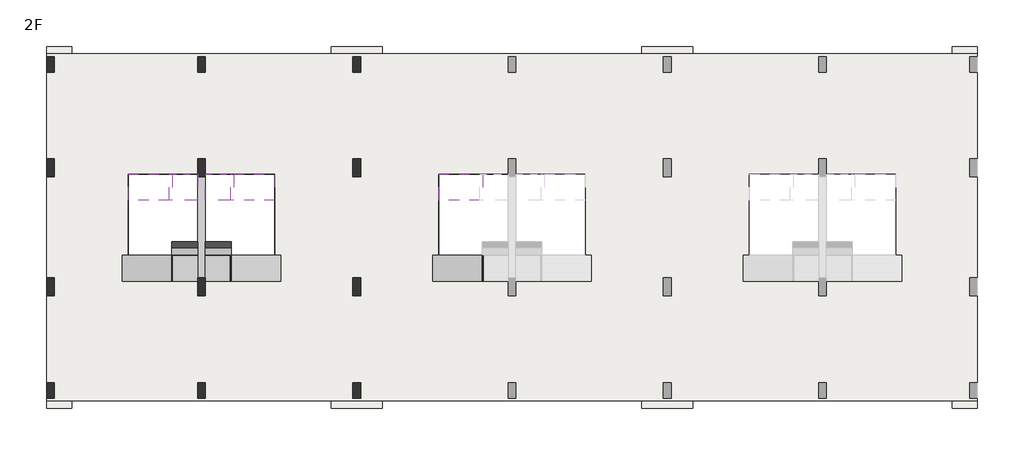
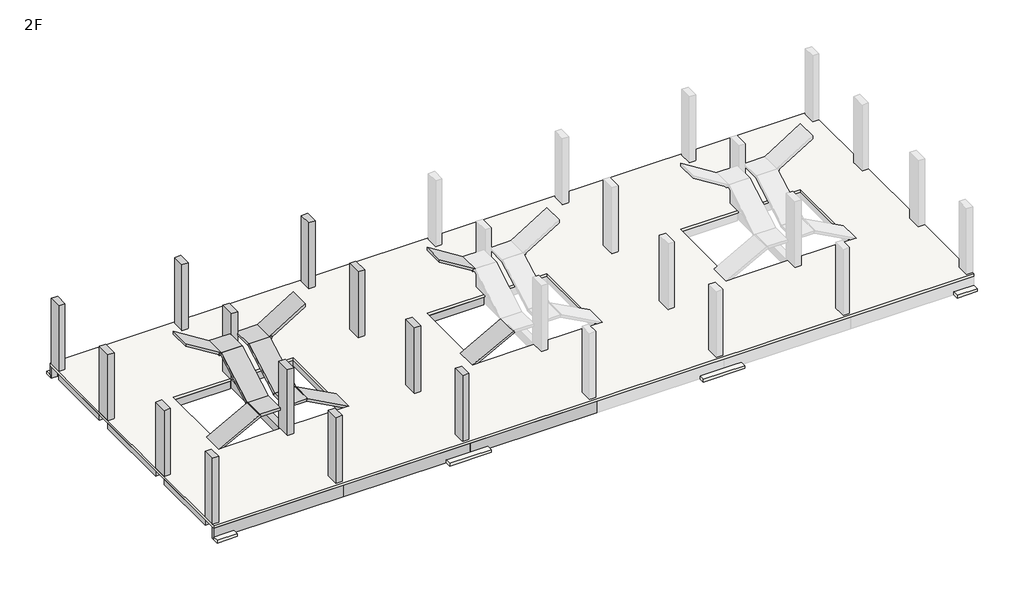
# One storey, part 1 of 2: 36 beams, 12 columns, 2 slabs.
"""IFC4 building model written with IfcOpenShell, lengths in millimetres."""

from ifc_helpers import new_model, si_unit, frame, origin, place, context, project, spatial, polyline, outline, extrude, faceted_brep, element, save

model = new_model("IFC4")

# Units and contexts
model_context = context("Model", 3, world=origin())
ifc_project = project(units=[si_unit("LENGTHUNIT", "METRE", prefix="MILLI")], contexts=[model_context])

# Site, building, storey
site = spatial("IfcSite", under=ifc_project)
building = spatial("IfcBuilding", under=site)
storey = spatial("IfcBuildingStorey", under=building, Name="2F", Elevation=4030.0)

# Beams
placement = place(None, origin())
element("IfcBeam", 1, ObjectType="M_Concrete-Rectangular Beam : 1000x120", at=placement, inside=storey, context=model_context, shape_type="Brep", body=[
    faceted_brep([(4730.4772067, 5424.9999998, 5080.0), (4730.4772067, 4424.9999998, 5080.0), (4787.1330577, 4424.9999998, 4974.2166623), (4787.1330577, 5424.9999998, 4974.2166623), (4700.0000007, 5424.9999998, 5063.6768996), (2770.0, 5424.9999998, 4030.0), (2770.0, 4424.9999998, 4030.0), (4700.0000007, 4424.9999998, 5063.6768996), (3024.1661582, 4424.9999998, 4030.0), (4760.5888269, 4424.9999998, 4960.0), (3024.1661582, 4449.9999998, 4030.0), (3020.0, 4449.9999998, 4027.7686728), (3020.0, 5424.9999998, 4027.7686728), (4760.5888269, 5424.9999998, 4960.0), (3020.0, 5424.9999998, 4030.0), (3020.0, 4449.9999998, 4030.0)], [[[0, 1, 2, 3]], [[1, 0, 4, 5, 6, 7]], [[2, 1, 7, 6, 8, 9]], [[3, 2, 9, 8, 10, 11, 12, 13]], [[0, 3, 13, 12, 14, 5, 4]], [[5, 14, 15, 10, 8, 6]], [[14, 12, 11, 15]], [[10, 15, 11]]]),
])
element("IfcBeam", 2, ObjectType="M_Concrete-Rectangular Beam : 1000x120", at=placement, inside=storey, context=model_context, shape_type="Brep", body=[
    faceted_brep([(4700.0000007, 7550.0000002, 6280.0), (5700.0000007, 7550.0000002, 6280.0), (5700.0000007, 7609.0063595, 6175.5095719), (4700.0000007, 7609.0063595, 6175.5095719), (4700.0000007, 5424.9999998, 5080.0), (4700.0000007, 5484.0063591, 4975.5095719), (5700.0000007, 5484.0063591, 4975.5095719), (5700.0000007, 5424.9999998, 5080.0), (5700.0000007, 5524.9999998, 4998.6589219), (5700.0000007, 7581.5414925, 6160.0), (4700.0000007, 5524.9999998, 4998.6589219), (4700.0000007, 7581.5414925, 6160.0)], [[[0, 1, 2, 3]], [[4, 5, 6, 7]], [[1, 0, 4, 7]], [[2, 1, 7, 6, 8, 9]], [[3, 2, 9, 8, 6, 5, 10, 11]], [[0, 3, 11, 10, 5, 4]]]),
])
element("IfcBeam", 3, ObjectType="M_Concrete-Rectangular Beam : 1000x120", at=placement, inside=storey, context=model_context, shape_type="Brep", body=[
    faceted_brep([(4600.0000007, 7550.0000002, 6280.0), (4600.0000007, 8550.0000002, 6280.0), (4600.0000007, 8550.0000002, 6160.0), (4600.0000007, 7550.0000002, 6160.0), (5700.0000007, 8550.0000002, 6160.0), (5700.0000007, 8550.0000002, 6280.0), (5700.0000007, 7550.0000002, 6280.0), (5700.0000007, 7609.0063595, 6175.5095719), (5700.0000007, 7581.5414925, 6160.0), (4700.0000007, 7550.0000002, 6280.0), (4700.0000007, 7581.5414925, 6160.0), (4700.0000007, 7550.0000002, 6160.0), (4700.0000007, 7609.0063595, 6175.5095719)], [[[0, 1, 2, 3]], [[4, 5, 6, 7, 8]], [[1, 0, 9, 6, 5]], [[2, 1, 5, 4]], [[3, 2, 4, 8, 10, 11]], [[0, 3, 11, 9]], [[12, 7, 6, 9]], [[7, 12, 10, 8]], [[12, 9, 11, 10]]]),
])
element("IfcBeam", 4, ObjectType="M_Concrete-Rectangular Beam : 1000x120", at=placement, inside=storey, context=model_context, shape_type="Brep", body=[
    faceted_brep([(3019.99996, 7549.9999993, 7330.0), (4715.7503089, 7549.9999993, 6280.0), (4715.7503089, 8549.9999993, 6280.0), (3019.99996, 8549.9999993, 7330.0), (4600.0000007, 8549.9999993, 6280.0), (4600.0000007, 8549.9999993, 6210.5302519), (3020.0, 8549.9999993, 7188.8582245), (4600.0000007, 7549.9999993, 6210.5302519), (3020.0, 7549.9999993, 7188.8582245), (4600.0000007, 7549.9999993, 6280.0), (4700.0000007, 7549.9999993, 6280.0)], [[[0, 1, 2, 3]], [[3, 2, 4, 5, 6]], [[5, 7, 8, 6]], [[1, 0, 8, 7, 9, 10]], [[4, 9, 7, 5]], [[9, 4, 2, 1, 10]], [[0, 3, 6, 8]]]),
])
element("IfcBeam", 5, ObjectType="M_Concrete-Rectangular Beam : 1000x120", at=placement, inside=storey, context=model_context, shape_type="Brep", body=[
    faceted_brep([(5700.0000007, 5524.9999998, 4960.0), (4700.0000007, 5524.9999998, 4960.0), (4700.0000007, 5524.9999998, 4998.6589219), (5700.0000007, 5524.9999998, 4998.6589219), (5700.0000007, 4424.9999998, 4960.0), (5700.0000007, 4424.9999998, 5080.0), (4730.4772067, 4424.9999998, 5080.0), (4787.1330577, 4424.9999998, 4974.2166623), (4760.5888269, 4424.9999998, 4960.0), (5700.0000007, 5424.9999998, 5080.0), (4700.0000007, 5424.9999998, 5080.0), (4700.0000007, 4424.9999998, 5080.0), (5700.0000007, 5484.0063591, 4975.5095719), (4760.5888269, 5424.9999998, 4960.0), (4700.0000007, 5424.9999998, 4960.0), (4700.0000007, 4424.9999998, 5063.6768996), (4700.0000007, 5484.0063591, 4975.5095719), (4700.0000007, 5424.9999998, 5063.6768996), (4730.4772067, 5424.9999998, 5080.0), (4787.1330577, 5424.9999998, 4974.2166623)], [[[0, 1, 2, 3]], [[4, 5, 6, 7, 8]], [[6, 5, 9, 10, 11]], [[5, 4, 0, 3, 12, 9]], [[1, 0, 4, 8, 13, 14]], [[15, 11, 10, 16, 2, 1, 14, 17]], [[6, 18, 19, 7]], [[18, 6, 15, 17]], [[7, 19, 13, 8]], [[19, 18, 17, 14, 13]], [[11, 15, 6]], [[12, 16, 10, 9]], [[16, 12, 3, 2]]]),
])
element("IfcBeam", 6, ObjectType="M_Concrete-Rectangular Beam : 1000x120", at=placement, inside=storey, context=model_context, shape_type="Brep", body=[
    faceted_brep([(6969.5227948, 4424.9999998, 5080.0), (6969.5227948, 5424.9999998, 5080.0), (6912.8669437, 5424.9999998, 4974.2166623), (6912.8669437, 4424.9999998, 4974.2166623), (7000.0000007, 4424.9999998, 5063.6768996), (8930.0000014, 4424.9999998, 4030.0), (8930.0000014, 5424.9999998, 4030.0), (7000.0000007, 5424.9999998, 5063.6768996), (6939.4111745, 4424.9999998, 4960.0), (8675.8338433, 4424.9999998, 4030.0), (6939.4111745, 5424.9999998, 4960.0), (8680.0, 5424.9999998, 4027.7686736), (8680.0, 4449.9999998, 4027.7686736), (8675.8338433, 4449.9999998, 4030.0), (8680.0, 5424.9999998, 4030.0), (8680.0, 4449.9999998, 4030.0)], [[[0, 1, 2, 3]], [[1, 0, 4, 5, 6, 7]], [[0, 3, 8, 9, 5, 4]], [[3, 2, 10, 11, 12, 13, 9, 8]], [[2, 1, 7, 6, 14, 11, 10]], [[14, 6, 5, 9, 13, 15]], [[11, 14, 15, 12]], [[15, 13, 12]]]),
])
element("IfcBeam", 7, ObjectType="M_Concrete-Rectangular Beam : 1000x120", at=placement, inside=storey, context=model_context, shape_type="Brep", body=[
    faceted_brep([(7000.0000007, 7550.0000002, 6280.0), (7000.0000007, 7609.0063595, 6175.5095719), (6000.0000007, 7609.0063595, 6175.5095719), (6000.0000007, 7550.0000002, 6280.0), (7000.0000007, 5424.9999998, 5080.0), (6000.0000007, 5424.9999998, 5080.0), (6000.0000007, 5484.0063591, 4975.5095719), (7000.0000007, 5484.0063591, 4975.5095719), (6000.0000007, 7581.5414925, 6160.0), (6000.0000007, 5524.9999998, 4998.6589219), (7000.0000007, 7581.5414925, 6160.0), (7000.0000007, 5524.9999998, 4998.6589219)], [[[0, 1, 2, 3]], [[4, 5, 6, 7]], [[3, 5, 4, 0]], [[2, 8, 9, 6, 5, 3]], [[1, 10, 11, 7, 6, 9, 8, 2]], [[0, 4, 7, 11, 10, 1]]]),
])
element("IfcBeam", 8, ObjectType="M_Concrete-Rectangular Beam : 1000x120", at=placement, inside=storey, context=model_context, shape_type="Brep", body=[
    faceted_brep([(7100.0000007, 8550.0000002, 6280.0), (7100.0000007, 7550.0000002, 6280.0), (7100.0000007, 7550.0000002, 6160.0), (7100.0000007, 8550.0000002, 6160.0), (6000.0000007, 8550.0000002, 6280.0), (6000.0000007, 8550.0000002, 6160.0), (6000.0000007, 7581.5414925, 6160.0), (6000.0000007, 7609.0063595, 6175.5095719), (6000.0000007, 7550.0000002, 6280.0), (7000.0000007, 7550.0000002, 6280.0), (7000.0000007, 7550.0000002, 6160.0), (7000.0000007, 7581.5414925, 6160.0), (7000.0000007, 7609.0063595, 6175.5095719)], [[[0, 1, 2, 3]], [[4, 5, 6, 7, 8]], [[1, 0, 4, 8, 9]], [[0, 3, 5, 4]], [[3, 2, 10, 11, 6, 5]], [[2, 1, 9, 10]], [[12, 9, 8, 7]], [[12, 7, 6, 11]], [[9, 12, 11, 10]]]),
])
element("IfcBeam", 9, ObjectType="M_Concrete-Rectangular Beam : 1000x120", at=placement, inside=storey, context=model_context, shape_type="Brep", body=[
    faceted_brep([(6984.2496926, 7549.9999993, 6280.0), (8680.0000414, 7549.9999993, 7330.0), (8680.0, 8549.9999993, 7329.9999744), (6984.2496926, 8549.9999993, 6280.0), (8680.0, 8549.9999993, 7188.8582236), (7100.0000007, 8549.9999993, 6210.5302519), (7100.0000007, 8549.9999993, 6280.0), (7100.0000007, 7549.9999993, 6210.5302519), (8680.0, 7549.9999993, 7188.8582236), (7000.0000007, 7549.9999993, 6280.0), (7100.0000007, 7549.9999993, 6280.0)], [[[0, 1, 2, 3]], [[3, 2, 4, 5, 6]], [[7, 5, 4, 8]], [[1, 0, 9, 10, 7, 8]], [[10, 6, 5, 7]], [[6, 10, 9, 0, 3]], [[2, 1, 8, 4]]]),
])
element("IfcBeam", 10, ObjectType="M_Concrete-Rectangular Beam : 1000x120", at=placement, inside=storey, context=model_context, shape_type="Brep", body=[
    faceted_brep([(7000.0000007, 5524.9999998, 4960.0), (6000.0000007, 5524.9999998, 4960.0), (6000.0000007, 5524.9999998, 4998.6589219), (7000.0000007, 5524.9999998, 4998.6589219), (6000.0000007, 4424.9999998, 5080.0), (6000.0000007, 4424.9999998, 4960.0), (6939.4111745, 4424.9999998, 4960.0), (6912.8669437, 4424.9999998, 4974.2166623), (6969.5227948, 4424.9999998, 5080.0), (7000.0000007, 4424.9999998, 5080.0), (7000.0000007, 5424.9999998, 5080.0), (6000.0000007, 5424.9999998, 5080.0), (6000.0000007, 5484.0063591, 4975.5095719), (7000.0000007, 5424.9999998, 4960.0), (6939.4111745, 5424.9999998, 4960.0), (7000.0000007, 4424.9999998, 5063.6768996), (7000.0000007, 5424.9999998, 5063.6768996), (7000.0000007, 5484.0063591, 4975.5095719), (6969.5227948, 5424.9999998, 5080.0), (6912.8669437, 5424.9999998, 4974.2166623)], [[[0, 1, 2, 3]], [[4, 5, 6, 7, 8]], [[8, 9, 10, 11, 4]], [[5, 4, 11, 12, 2, 1]], [[1, 0, 13, 14, 6, 5]], [[9, 15, 16, 13, 0, 3, 17, 10]], [[18, 8, 7, 19]], [[8, 18, 16, 15]], [[19, 7, 6, 14]], [[18, 19, 14, 13, 16]], [[15, 9, 8]], [[17, 12, 11, 10]], [[12, 17, 3, 2]]]),
])
element("IfcBeam", 11, ObjectType="M_Concrete-Rectangular Beam : 1000x120", at=placement, inside=storey, context=model_context, shape_type="Brep", body=[
    faceted_brep([(16730.4772117, 5424.9999998, 5080.0), (16730.4772117, 4424.9999998, 5080.0), (16787.1330628, 4424.9999998, 4974.2166623), (16787.1330628, 5424.9999998, 4974.2166623), (16700.0000058, 5424.9999998, 5063.6768996), (14770.000005, 5424.9999998, 4030.0), (14770.000005, 4424.9999998, 4030.0), (16700.0000058, 4424.9999998, 5063.6768996), (15024.1661632, 4424.9999998, 4030.0), (16760.588832, 4424.9999998, 4960.0), (15024.1661632, 4449.9999998, 4030.0), (15020.0000057, 4449.9999998, 4027.7686732), (15020.0000057, 5424.9999998, 4027.7686732), (16760.588832, 5424.9999998, 4960.0), (15020.0000057, 5424.9999998, 4030.0), (15020.0000057, 4449.9999998, 4030.0)], [[[0, 1, 2, 3]], [[1, 0, 4, 5, 6, 7]], [[2, 1, 7, 6, 8, 9]], [[3, 2, 9, 8, 10, 11, 12, 13]], [[0, 3, 13, 12, 14, 5, 4]], [[5, 14, 15, 10, 8, 6]], [[14, 12, 11, 15]], [[10, 15, 11]]]),
])
element("IfcBeam", 12, ObjectType="M_Concrete-Rectangular Beam : 1000x120", at=placement, inside=storey, context=model_context, shape_type="Brep", body=[
    faceted_brep([(15019.9999651, 7549.9999993, 7330.0), (16715.7503139, 7549.9999993, 6280.0), (16715.7503139, 8549.9999993, 6280.0), (15019.9999651, 8549.9999993, 7330.0), (16600.0000058, 8549.9999993, 6280.0), (16600.0000058, 8549.9999993, 6210.5302519), (15020.0000057, 8549.9999993, 7188.8582241), (16600.0000058, 7549.9999993, 6210.5302519), (15020.0000057, 7549.9999993, 7188.8582241), (16600.0000058, 7549.9999993, 6280.0), (16700.0000058, 7549.9999993, 6280.0)], [[[0, 1, 2, 3]], [[3, 2, 4, 5, 6]], [[5, 7, 8, 6]], [[1, 0, 8, 7, 9, 10]], [[4, 9, 7, 5]], [[9, 4, 2, 1, 10]], [[0, 3, 6, 8]]]),
])
element("IfcBeam", 13, ObjectType="M_Concrete-Rectangular Beam : 250x400", at=placement, inside=storey, context=model_context, shape_type="Brep", body=[
    faceted_brep([(8680.0, 8549.9999993, 3630.0), (8680.0, 4449.9999998, 3630.0), (8680.0, 4449.9999998, 3900.0), (8680.0, 8549.9999993, 3900.0), (8680.0, 8549.9999993, 3881.8224529), (8930.0, 8549.9999993, 3630.0), (8930.0, 4449.9999998, 3630.0), (8930.0, 8549.9999993, 3900.0), (8930.0, 4449.9999998, 3900.0)], [[[0, 1, 2, 3, 4]], [[0, 5, 6, 1]], [[6, 5, 7, 8]], [[5, 0, 4, 3, 7]], [[1, 6, 8, 2]], [[3, 2, 8, 7]]]),
])
element("IfcBeam", 14, ObjectType="M_Concrete-Rectangular Beam : 250x400", at=placement, inside=storey, context=model_context, shape_type="Brep", body=[
    faceted_brep([(15020.0000057, 4449.9999998, 3630.0), (15020.0000057, 8549.9999993, 3630.0), (15020.0000057, 8549.9999993, 3881.8224534), (15020.0000057, 8549.9999993, 3900.0), (15020.0000057, 4449.9999998, 3900.0), (14770.0000057, 8549.9999993, 3630.0), (14770.0000057, 4449.9999998, 3630.0), (14770.0000057, 4449.9999998, 3900.0), (14770.0000057, 8549.9999993, 3900.0)], [[[0, 1, 2, 3, 4]], [[5, 1, 0, 6]], [[5, 6, 7, 8]], [[1, 5, 8, 3, 2]], [[6, 0, 4, 7]], [[4, 3, 8, 7]]]),
])
element("IfcBeam", 15, ObjectType="M_Concrete-Rectangular Beam : 250x400", at=placement, inside=storey, context=model_context, shape_type="Brep", body=[
    faceted_brep([(3020.0, 4449.9999998, 3630.0), (3020.0, 8549.9999993, 3630.0), (3020.0, 8549.9999993, 3881.8224539), (3020.0, 8549.9999993, 3900.0), (3020.0, 4449.9999998, 3900.0), (2770.0, 8549.9999993, 3630.0), (2770.0, 4449.9999998, 3630.0), (2770.0, 4449.9999998, 3900.0), (2770.0, 8549.9999993, 3900.0)], [[[0, 1, 2, 3, 4]], [[5, 1, 0, 6]], [[5, 6, 7, 8]], [[1, 5, 8, 3, 2]], [[6, 0, 4, 7]], [[4, 3, 8, 7]]]),
])
element("IfcBeam", 16, ObjectType="M_Concrete-Rectangular Beam : 300x400", at=placement, inside=storey, context=model_context, shape_type="SweptSolid", body=[
    extrude(outline(polyline([(165.0, 9149.9985388), (-135.0, 9149.9985388), (-135.0, 12500.0000003), (165.0, 12500.0000003), (165.0, 9149.9985388)])), frame((0.0, 0.0, 3630.0), z_axis=(0.0, 0.0, 1.0), x_axis=(1.0, 0.0, 0.0)), (0.0, 0.0, 1.0), 270.0),
])
element("IfcBeam", 17, ObjectType="M_Concrete-Rectangular Beam : 300x400", at=placement, inside=storey, context=model_context, shape_type="SweptSolid", body=[
    extrude(outline(polyline([(165.0, 4550.0000002), (-135.0, 4550.0000002), (-135.0, 8449.9985388), (165.0, 8449.9985388), (165.0, 4550.0000002)])), frame((0.0, 0.0, 3630.0), z_axis=(0.0, 0.0, 1.0), x_axis=(1.0, 0.0, 0.0)), (0.0, 0.0, 1.0), 270.0),
])
element("IfcBeam", 18, ObjectType="M_Concrete-Rectangular Beam : 300x400", at=placement, inside=storey, context=model_context, shape_type="SweptSolid", body=[
    extrude(outline(polyline([(165.0, 499.9999998), (-135.0, 499.9999998), (-135.0, 3850.0000002), (165.0, 3850.0000002), (165.0, 499.9999998)])), frame((0.0, 0.0, 3630.0), z_axis=(0.0, 0.0, 1.0), x_axis=(1.0, 0.0, 0.0)), (0.0, 0.0, 1.0), 270.0),
])
element("IfcBeam", 19, ObjectType="M_Concrete-Rectangular Beam : 300x400", at=placement, inside=storey, context=model_context, shape_type="SweptSolid", body=[
    extrude(outline(polyline([(12000.0000027, 4550.0000002), (11700.0000027, 4550.0000002), (11700.0000027, 8449.9985388), (12000.0000027, 8449.9985388), (12000.0000027, 4550.0000002)])), frame((0.0, 0.0, 3630.0), z_axis=(0.0, 0.0, 1.0), x_axis=(1.0, 0.0, 0.0)), (0.0, 0.0, 1.0), 270.0),
])
element("IfcBeam", 20, ObjectType="M_Concrete-Rectangular Beam : 300x400", at=placement, inside=storey, context=model_context, shape_type="SweptSolid", body=[
    extrude(outline(polyline([(6000.0, 4550.0000002), (5700.0, 4550.0000002), (5700.0, 8449.9985388), (6000.0, 8449.9985388), (6000.0, 4550.0000002)])), frame((0.0, 0.0, 3630.0), z_axis=(0.0, 0.0, 1.0), x_axis=(1.0, 0.0, 0.0)), (0.0, 0.0, 1.0), 400.0),
])
element("IfcBeam", 21, ObjectType="M_Concrete-Rectangular Beam : 300x400", at=placement, inside=storey, context=model_context, shape_type="SweptSolid", body=[
    extrude(outline(polyline([(6000.0000007, 499.9999998), (5700.0000007, 499.9999998), (5700.0000007, 3850.0000002), (6000.0000007, 3850.0000002), (6000.0000007, 499.9999998)])), frame((0.0, 0.0, 3630.0), z_axis=(0.0, 0.0, 1.0), x_axis=(1.0, 0.0, 0.0)), (0.0, 0.0, 1.0), 270.0),
])
element("IfcBeam", 22, ObjectType="M_Concrete-Rectangular Beam : 300x400", at=placement, inside=storey, context=model_context, shape_type="SweptSolid", body=[
    extrude(outline(polyline([(6000.0000007, 9149.9985388), (5700.0000007, 9149.9985388), (5700.0000007, 12500.0000003), (6000.0000007, 12500.0000003), (6000.0000007, 9149.9985388)])), frame((0.0, 0.0, 3630.0), z_axis=(0.0, 0.0, 1.0), x_axis=(1.0, 0.0, 0.0)), (0.0, 0.0, 1.0), 270.0),
])
element("IfcBeam", 23, ObjectType="M_Concrete-Rectangular Beam : 300x400", at=placement, inside=storey, context=model_context, shape_type="SweptSolid", body=[
    extrude(outline(polyline([(12000.0000034, 499.9999998), (11700.0000034, 499.9999998), (11700.0000034, 3850.0000002), (12000.0000034, 3850.0000002), (12000.0000034, 499.9999998)])), frame((0.0, 0.0, 3630.0), z_axis=(0.0, 0.0, 1.0), x_axis=(1.0, 0.0, 0.0)), (0.0, 0.0, 1.0), 270.0),
])
element("IfcBeam", 24, ObjectType="M_Concrete-Rectangular Beam : 300x400", at=placement, inside=storey, context=model_context, shape_type="SweptSolid", body=[
    extrude(outline(polyline([(12000.0000034, 9149.9985388), (11700.0000034, 9149.9985388), (11700.0000034, 12500.0000003), (12000.0000034, 12500.0000003), (12000.0000034, 9149.9985388)])), frame((0.0, 0.0, 3630.0), z_axis=(0.0, 0.0, 1.0), x_axis=(1.0, 0.0, 0.0)), (0.0, 0.0, 1.0), 270.0),
])
element("IfcBeam", 25, ObjectType="M_Concrete-Rectangular Beam : 300x500", at=placement, inside=storey, context=model_context, shape_type="Brep", body=[
    faceted_brep([(165.0, 8549.9999993, 3530.0), (5700.0000007, 8549.9999993, 3530.0), (5700.0000007, 8549.9999993, 3900.0), (3020.0, 8549.9999993, 3900.0), (2770.0, 8549.9999993, 3900.0), (165.0, 8549.9999993, 3900.0), (165.0, 8849.9999993, 3530.0), (5700.0000007, 8849.9999993, 3530.0), (165.0, 8849.9999993, 3900.0), (5700.0000007, 8849.9999993, 3900.0)], [[[0, 1, 2, 3, 4, 5]], [[0, 6, 7, 1]], [[7, 6, 8, 9]], [[6, 0, 5, 8]], [[1, 7, 9, 2]], [[5, 4, 3, 2, 9, 8]]]),
])
element("IfcBeam", 26, ObjectType="M_Concrete-Rectangular Beam : 300x500", at=placement, inside=storey, context=model_context, shape_type="Brep", body=[
    faceted_brep([(165.0, 4149.9999998, 3530.0), (5700.0000007, 4149.9999998, 3530.0), (5700.0000007, 4149.9999998, 3900.0), (165.0, 4149.9999998, 3900.0), (165.0, 4449.9999998, 3530.0), (5700.0000007, 4449.9999998, 3530.0), (165.0, 4449.9999998, 3900.0), (2770.0, 4449.9999998, 3900.0), (3020.0, 4449.9999998, 3900.0), (5700.0000007, 4449.9999998, 3900.0)], [[[0, 1, 2, 3]], [[0, 4, 5, 1]], [[5, 4, 6, 7, 8, 9]], [[4, 0, 3, 6]], [[1, 5, 9, 2]], [[3, 2, 9, 8, 7, 6]]]),
])
element("IfcBeam", 27, ObjectType="M_Concrete-Rectangular Beam : 300x500", at=placement, inside=storey, context=model_context, shape_type="Brep", body=[
    faceted_brep([(6000.0000007, 8549.9999993, 3530.0), (11700.0000034, 8549.9999993, 3530.0), (11700.0000034, 8549.9999993, 3900.0), (8930.0, 8549.9999993, 3900.0), (8680.0, 8549.9999993, 3900.0), (6000.0000002, 8549.9999993, 3900.0), (6000.0000007, 8849.9999993, 3530.0), (11700.0000034, 8849.9999993, 3530.0), (6000.0000007, 8849.9999993, 3900.0), (11700.0000034, 8849.9999993, 3900.0)], [[[0, 1, 2, 3, 4, 5]], [[0, 6, 7, 1]], [[7, 6, 8, 9]], [[6, 0, 5, 8]], [[1, 7, 9, 2]], [[5, 4, 3, 2, 9, 8]]]),
])
element("IfcBeam", 28, ObjectType="M_Concrete-Rectangular Beam : 300x500", at=placement, inside=storey, context=model_context, shape_type="Brep", body=[
    faceted_brep([(6000.0000007, 4149.9999998, 3530.0), (11700.0000034, 4149.9999998, 3530.0), (11700.0000034, 4149.9999998, 3900.0), (6000.0000007, 4149.9999998, 3900.0), (6000.0000007, 4449.9999998, 3530.0), (11700.0000034, 4449.9999998, 3530.0), (6000.0000002, 4449.9999998, 3900.0), (8680.0, 4449.9999998, 3900.0), (8930.0, 4449.9999998, 3900.0), (11700.0000034, 4449.9999998, 3900.0)], [[[0, 1, 2, 3]], [[0, 4, 5, 1]], [[5, 4, 6, 7, 8, 9]], [[4, 0, 3, 6]], [[1, 5, 9, 2]], [[3, 2, 9, 8, 7, 6]]]),
])
element("IfcBeam", 29, ObjectType="M_Concrete-Rectangular Beam : 300x500", at=placement, inside=storey, context=model_context, shape_type="Brep", body=[
    faceted_brep([(12000.0000034, 8549.9999993, 3530.0), (17700.0000058, 8549.9999993, 3530.0), (17700.0000058, 8549.9999993, 3900.0), (15020.0000057, 8549.9999993, 3900.0), (14770.0000057, 8549.9999993, 3900.0), (12000.0000029, 8549.9999993, 3900.0), (12000.0000034, 8849.9999993, 3530.0), (17700.0000058, 8849.9999993, 3530.0), (12000.0000034, 8849.9999993, 3900.0), (17700.0000058, 8849.9999993, 3900.0)], [[[0, 1, 2, 3, 4, 5]], [[0, 6, 7, 1]], [[7, 6, 8, 9]], [[6, 0, 5, 8]], [[1, 7, 9, 2]], [[5, 4, 3, 2, 9, 8]]]),
])
element("IfcBeam", 30, ObjectType="M_Concrete-Rectangular Beam : 300x500", at=placement, inside=storey, context=model_context, shape_type="Brep", body=[
    faceted_brep([(12000.0000034, 4149.9999998, 3530.0), (17700.0000058, 4149.9999998, 3530.0), (17700.0000058, 4149.9999998, 3900.0), (12000.0000034, 4149.9999998, 3900.0), (12000.0000034, 4449.9999998, 3530.0), (17700.0000058, 4449.9999998, 3530.0), (12000.0000029, 4449.9999998, 3900.0), (14770.0000057, 4449.9999998, 3900.0), (15020.0000057, 4449.9999998, 3900.0), (17700.0000058, 4449.9999998, 3900.0)], [[[0, 1, 2, 3]], [[0, 4, 5, 1]], [[5, 4, 6, 7, 8, 9]], [[4, 0, 3, 6]], [[1, 5, 9, 2]], [[3, 2, 9, 8, 7, 6]]]),
])
element("IfcBeam", 31, ObjectType="M_Concrete-Rectangular Beam : 400x700", at=placement, inside=storey, context=model_context, shape_type="Brep", body=[
    faceted_brep([(164.9999993, 12799.9999993, 3330.0), (5700.0000007, 12799.9999993, 3330.0), (5700.0000007, 12799.9999993, 3900.0), (164.9999993, 12799.9999993, 3900.0), (164.9999993, 13100.0000003, 3330.0), (-135.0, 13100.0000003, 3330.0), (-135.0, 13199.9999993, 3330.0), (830.0, 13199.9999993, 3330.0), (6000.0000007, 13199.9999993, 3330.0), (6000.0000007, 13100.0000003, 3330.0), (5700.0000007, 13100.0000003, 3330.0), (6000.0000007, 13199.9999993, 3900.0), (-135.0, 13199.9999993, 3460.0), (-135.0, 13199.9999993, 3900.0), (164.9999993, 13100.0000003, 3900.0), (-135.0, 13100.0000003, 3900.0), (5700.0000007, 13100.0000003, 3900.0), (6000.0000007, 13100.0000003, 3900.0)], [[[0, 1, 2, 3]], [[0, 4, 5, 6, 7, 8, 9, 10, 1]], [[11, 8, 7, 6, 12, 13]], [[4, 0, 3, 14]], [[5, 4, 14, 15]], [[1, 10, 16, 2]], [[10, 9, 17, 16]], [[6, 5, 15, 13, 12]], [[9, 8, 11, 17]], [[3, 2, 16, 17, 11, 13, 15, 14]]]),
])
element("IfcBeam", 32, ObjectType="M_Concrete-Rectangular Beam : 400x700", at=placement, inside=storey, context=model_context, shape_type="Brep", body=[
    faceted_brep([(6000.0000007, -199.999999, 3330.0), (6000.0000007, -199.999999, 3900.0), (-135.0, -199.999999, 3900.0), (-135.0, -199.999999, 3460.0), (-135.0, -199.999999, 3330.0), (830.0, -199.999999, 3330.0), (165.0, -100.0000002, 3330.0), (165.0, 200.000001, 3330.0), (5700.0000007, 200.000001, 3330.0), (5700.0000007, -100.0000002, 3330.0), (6000.0000007, -100.0000002, 3330.0), (-135.0, -100.0000002, 3330.0), (165.0, 200.000001, 3900.0), (5700.0000007, 200.000001, 3900.0), (165.0, -100.0000002, 3900.0), (-135.0, -100.0000002, 3900.0), (5700.0000007, -100.0000002, 3900.0), (6000.0000007, -100.0000002, 3900.0)], [[[0, 1, 2, 3, 4, 5]], [[6, 7, 8, 9, 10, 0, 5, 4, 11]], [[8, 7, 12, 13]], [[7, 6, 14, 12]], [[6, 11, 15, 14]], [[10, 9, 16, 17]], [[9, 8, 13, 16]], [[11, 4, 3, 2, 15]], [[0, 10, 17, 1]], [[2, 1, 17, 16, 13, 12, 14, 15]]]),
])
element("IfcBeam", 33, ObjectType="M_Concrete-Rectangular Beam : 400x700", at=placement, inside=storey, context=model_context, shape_type="Brep", body=[
    faceted_brep([(6000.0000007, 12799.9999993, 3330.0), (11700.0000034, 12799.9999993, 3330.0), (11700.0000034, 12799.9999993, 3900.0), (6000.0000007, 12799.9999993, 3900.0), (11700.0000034, 13100.0000003, 3330.0), (6000.0000007, 13100.0000003, 3330.0), (6000.0000007, 13199.9999993, 3330.0), (10870.0000007, 13199.9999993, 3330.0), (12000.0000034, 13199.9999993, 3330.0), (12000.0000034, 13100.0000003, 3330.0), (6000.0000007, 13199.9999993, 3900.0), (12000.0000034, 13199.9999993, 3900.0), (12000.0000034, 13199.9999993, 3460.0), (11700.0000034, 13100.0000003, 3900.0), (12000.0000034, 13100.0000003, 3900.0), (6000.0000007, 13100.0000003, 3900.0)], [[[0, 1, 2, 3]], [[4, 1, 0, 5, 6, 7, 8, 9]], [[6, 10, 11, 12, 8, 7]], [[1, 4, 13, 2]], [[4, 9, 14, 13]], [[9, 8, 12, 11, 14]], [[6, 5, 0, 3, 15, 10]], [[3, 2, 13, 14, 11, 10, 15]]]),
])
element("IfcBeam", 34, ObjectType="M_Concrete-Rectangular Beam : 400x700", at=placement, inside=storey, context=model_context, shape_type="Brep", body=[
    faceted_brep([(6000.0000007, -199.999999, 3900.0), (6000.0000007, -199.999999, 3330.0), (10870.0000007, -199.999999, 3330.0), (12000.0000034, -199.999999, 3330.0), (12000.0000034, -199.999999, 3460.0), (12000.0000034, -199.999999, 3900.0), (11700.0000034, -100.0000002, 3330.0), (12000.0000034, -100.0000002, 3330.0), (6000.0000007, -100.0000002, 3330.0), (6000.0000007, 200.000001, 3330.0), (11700.0000034, 200.000001, 3330.0), (6000.0000007, 200.000001, 3900.0), (11700.0000034, 200.000001, 3900.0), (11700.0000034, -100.0000002, 3900.0), (12000.0000034, -100.0000002, 3900.0), (6000.0000007, -100.0000002, 3900.0)], [[[0, 1, 2, 3, 4, 5]], [[6, 7, 3, 2, 1, 8, 9, 10]], [[10, 9, 11, 12]], [[7, 6, 13, 14]], [[6, 10, 12, 13]], [[3, 7, 14, 5, 4]], [[9, 8, 1, 0, 15, 11]], [[0, 5, 14, 13, 12, 11, 15]]]),
])
element("IfcBeam", 35, ObjectType="M_Concrete-Rectangular Beam : 400x700", at=placement, inside=storey, context=model_context, shape_type="Brep", body=[
    faceted_brep([(12000.0000034, 12799.9999993, 3330.0), (17700.0000058, 12799.9999993, 3330.0), (17700.0000058, 12799.9999993, 3900.0), (12000.0000034, 12799.9999993, 3900.0), (17700.0000058, 13100.0000003, 3330.0), (12000.0000034, 13100.0000003, 3330.0), (12000.0000034, 13199.9999993, 3330.0), (12829.7667679, 13199.9999993, 3330.0), (18000.0000046, 13199.9999993, 3330.0), (18000.0000046, 13100.0000003, 3330.0), (18000.0000046, 13199.9999993, 3900.0), (12000.0000034, 13199.9999993, 3460.0), (12000.0000034, 13199.9999993, 3900.0), (17700.0000058, 13100.0000003, 3900.0), (18000.0000046, 13100.0000003, 3900.0), (12000.0000034, 13100.0000003, 3900.0)], [[[0, 1, 2, 3]], [[4, 1, 0, 5, 6, 7, 8, 9]], [[10, 8, 7, 6, 11, 12]], [[1, 4, 13, 2]], [[4, 9, 14, 13]], [[9, 8, 10, 14]], [[6, 5, 0, 3, 15, 12, 11]], [[3, 2, 13, 14, 10, 12, 15]]]),
])
element("IfcBeam", 36, ObjectType="M_Concrete-Rectangular Beam : 400x700", at=placement, inside=storey, context=model_context, shape_type="Brep", body=[
    faceted_brep([(18000.0000046, -199.999999, 3330.0), (18000.0000046, -199.999999, 3900.0), (12000.0000034, -199.999999, 3900.0), (12000.0000034, -199.999999, 3460.0), (12000.0000034, -199.999999, 3330.0), (12830.0000047, -199.999999, 3330.0), (17700.0000058, -100.0000002, 3330.0), (18000.0000046, -100.0000002, 3330.0), (12000.0000034, -100.0000002, 3330.0), (12000.0000034, 200.000001, 3330.0), (17700.0000058, 200.000001, 3330.0), (12000.0000034, 200.000001, 3900.0), (17700.0000058, 200.000001, 3900.0), (17700.0000058, -100.0000002, 3900.0), (18000.0000046, -100.0000002, 3900.0), (12000.0000034, -100.0000002, 3900.0)], [[[0, 1, 2, 3, 4, 5]], [[6, 7, 0, 5, 4, 8, 9, 10]], [[10, 9, 11, 12]], [[7, 6, 13, 14]], [[6, 10, 12, 13]], [[0, 7, 14, 1]], [[9, 8, 4, 3, 2, 15, 11]], [[2, 1, 14, 13, 12, 11, 15]]]),
])

# Columns
element("IfcColumn", 37, ObjectType="M_Concrete-Rectangular-Column : 300x600", at=placement, inside=storey, context=model_context, shape_type="SweptSolid", body=[
    extrude(outline(polyline([(165.0, 499.9999998), (165.0, -100.0000002), (-135.0, -100.0000002), (-135.0, 499.9999998), (165.0, 499.9999998)])), frame((0.0, 0.0, 4030.0), z_axis=(0.0, 0.0, 1.0), x_axis=(1.0, 0.0, 0.0)), (0.0, 0.0, 1.0), 3300.0),
])
element("IfcColumn", 38, ObjectType="M_Concrete-Rectangular-Column : 300x600", at=placement, inside=storey, context=model_context, shape_type="SweptSolid", body=[
    extrude(outline(polyline([(164.9999993, 13100.0000003), (164.9999993, 12500.0000003), (-135.0000007, 12500.0000003), (-135.0000007, 13100.0000003), (164.9999993, 13100.0000003)])), frame((0.0, 0.0, 4030.0), z_axis=(0.0, 0.0, 1.0), x_axis=(1.0, 0.0, 0.0)), (0.0, 0.0, 1.0), 3300.0),
])
element("IfcColumn", 39, ObjectType="M_Concrete-Rectangular-Column : 300x600", at=placement, inside=storey, context=model_context, shape_type="SweptSolid", body=[
    extrude(outline(polyline([(6000.0000007, 499.9999998), (6000.0000007, -100.0000002), (5700.0000007, -100.0000002), (5700.0000007, 499.9999998), (6000.0000007, 499.9999998)])), frame((0.0, 0.0, 4030.0), z_axis=(0.0, 0.0, 1.0), x_axis=(1.0, 0.0, 0.0)), (0.0, 0.0, 1.0), 3300.0),
])
element("IfcColumn", 40, ObjectType="M_Concrete-Rectangular-Column : 300x600", at=placement, inside=storey, context=model_context, shape_type="SweptSolid", body=[
    extrude(outline(polyline([(12000.0000034, 499.9999998), (12000.0000034, -100.0000002), (11700.0000034, -100.0000002), (11700.0000034, 499.9999998), (12000.0000034, 499.9999998)])), frame((0.0, 0.0, 4030.0), z_axis=(0.0, 0.0, 1.0), x_axis=(1.0, 0.0, 0.0)), (0.0, 0.0, 1.0), 3300.0),
])
element("IfcColumn", 41, ObjectType="M_Concrete-Rectangular-Column : 300x600", at=placement, inside=storey, context=model_context, shape_type="SweptSolid", body=[
    extrude(outline(polyline([(6000.0000007, 13100.0000003), (6000.0000007, 12500.0000003), (5700.0000007, 12500.0000003), (5700.0000007, 13100.0000003), (6000.0000007, 13100.0000003)])), frame((0.0, 0.0, 4030.0), z_axis=(0.0, 0.0, 1.0), x_axis=(1.0, 0.0, 0.0)), (0.0, 0.0, 1.0), 3300.0),
])
element("IfcColumn", 42, ObjectType="M_Concrete-Rectangular-Column : 300x600", at=placement, inside=storey, context=model_context, shape_type="SweptSolid", body=[
    extrude(outline(polyline([(12000.0000034, 13100.0000003), (12000.0000034, 12500.0000003), (11700.0000034, 12500.0000003), (11700.0000034, 13100.0000003), (12000.0000034, 13100.0000003)])), frame((0.0, 0.0, 4030.0), z_axis=(0.0, 0.0, 1.0), x_axis=(1.0, 0.0, 0.0)), (0.0, 0.0, 1.0), 3300.0),
])
element("IfcColumn", 43, ObjectType="M_Concrete-Rectangular-Column : 300x700", at=placement, inside=storey, context=model_context, shape_type="SweptSolid", body=[
    extrude(outline(polyline([(165.0, 4550.0000002), (165.0, 3850.0000002), (-135.0, 3850.0000002), (-135.0, 4550.0000002), (165.0, 4550.0000002)])), frame((0.0, 0.0, 4030.0), z_axis=(0.0, 0.0, 1.0), x_axis=(1.0, 0.0, 0.0)), (0.0, 0.0, 1.0), 3300.0),
])
element("IfcColumn", 44, ObjectType="M_Concrete-Rectangular-Column : 300x700", at=placement, inside=storey, context=model_context, shape_type="SweptSolid", body=[
    extrude(outline(polyline([(165.0, 9149.9985388), (165.0, 8449.9985388), (-135.0, 8449.9985388), (-135.0, 9149.9985388), (165.0, 9149.9985388)])), frame((0.0, 0.0, 4030.0), z_axis=(0.0, 0.0, 1.0), x_axis=(1.0, 0.0, 0.0)), (0.0, 0.0, 1.0), 3300.0),
])
element("IfcColumn", 45, ObjectType="M_Concrete-Rectangular-Column : 300x700", at=placement, inside=storey, context=model_context, shape_type="SweptSolid", body=[
    extrude(outline(polyline([(6000.0000007, 4550.0000002), (6000.0000007, 3850.0000002), (5700.0000007, 3850.0000002), (5700.0000007, 4550.0000002), (6000.0000007, 4550.0000002)])), frame((0.0, 0.0, 4030.0), z_axis=(0.0, 0.0, 1.0), x_axis=(1.0, 0.0, 0.0)), (0.0, 0.0, 1.0), 3300.0),
])
element("IfcColumn", 46, ObjectType="M_Concrete-Rectangular-Column : 300x700", at=placement, inside=storey, context=model_context, shape_type="SweptSolid", body=[
    extrude(outline(polyline([(12000.0000034, 4550.0000002), (12000.0000034, 3850.0000002), (11700.0000034, 3850.0000002), (11700.0000034, 4550.0000002), (12000.0000034, 4550.0000002)])), frame((0.0, 0.0, 4030.0), z_axis=(0.0, 0.0, 1.0), x_axis=(1.0, 0.0, 0.0)), (0.0, 0.0, 1.0), 3300.0),
])
element("IfcColumn", 47, ObjectType="M_Concrete-Rectangular-Column : 300x700", at=placement, inside=storey, context=model_context, shape_type="SweptSolid", body=[
    extrude(outline(polyline([(6000.0000007, 9149.9985388), (6000.0000007, 8449.9985388), (5700.0000007, 8449.9985388), (5700.0000007, 9149.9985388), (6000.0000007, 9149.9985388)])), frame((0.0, 0.0, 4030.0), z_axis=(0.0, 0.0, 1.0), x_axis=(1.0, 0.0, 0.0)), (0.0, 0.0, 1.0), 3300.0),
])
element("IfcColumn", 48, ObjectType="M_Concrete-Rectangular-Column : 300x700", at=placement, inside=storey, context=model_context, shape_type="SweptSolid", body=[
    extrude(outline(polyline([(12000.0000034, 9149.9985388), (12000.0000034, 8449.9985388), (11700.0000034, 8449.9985388), (11700.0000034, 9149.9985388), (12000.0000034, 9149.9985388)])), frame((0.0, 0.0, 4030.0), z_axis=(0.0, 0.0, 1.0), x_axis=(1.0, 0.0, 0.0)), (0.0, 0.0, 1.0), 3300.0),
])

# Slabs
element("IfcSlab", 49, ObjectType="130", at=placement, inside=storey, context=model_context, shape_type="Brep", body=[
    faceted_brep([(35835.035019, 13199.9999993, 3900.0), (35835.035019, 13100.0000003, 3900.0), (35835.035019, 12500.0000003, 3900.0), (35835.035019, 9149.9985388, 3900.0), (35835.035019, 8449.9985388, 3900.0), (35835.035019, 4550.0000002, 3900.0), (35835.035019, 3850.0000002, 3900.0), (35835.035019, 499.9999998, 3900.0), (35835.035019, -100.0000002, 3900.0), (35835.035019, -199.999999, 3900.0), (30000.0000031, -199.999999, 3900.0), (24000.000004, -199.999999, 3900.0), (18000.0000046, -199.999999, 3900.0), (12000.0000034, -199.999999, 3900.0), (6000.0000007, -199.999999, 3900.0), (-135.0, -199.999999, 3900.0), (-135.0, -100.0000002, 3900.0), (-135.0, 499.9999998, 3900.0), (-135.0, 3850.0000002, 3900.0), (-135.0, 4550.0000002, 3900.0), (-135.0, 8449.9985388, 3900.0), (-135.0, 9149.9985388, 3900.0), (-135.0, 12500.0000003, 3900.0), (-135.0, 13100.0000003, 3900.0), (-135.0, 13199.9999993, 3900.0), (6000.0000007, 13199.9999993, 3900.0), (12000.0000034, 13199.9999993, 3900.0), (18000.0000046, 13199.9999993, 3900.0), (24000.000004, 13199.9999993, 3900.0), (30000.0000031, 13199.9999993, 3900.0), (8680.0, 4450.0000002, 3900.0), (8680.0, 8549.9999993, 3900.0), (6000.0000002, 8549.9999993, 3900.0), (5700.0000007, 8549.9999993, 3900.0), (3020.0, 8549.9999993, 3900.0), (3020.0, 4450.0000002, 3900.0), (5700.0000007, 4450.0000002, 3900.0), (6000.0000007, 4450.0000002, 3900.0), (32680.0000108, 4450.0000002, 3900.0), (32680.0000108, 8549.9999993, 3900.0), (30000.0000039, 8549.9999993, 3900.0), (29700.0000039, 8549.9999993, 3900.0), (27020.000004, 8549.9999993, 3900.0), (27020.000004, 4450.0000002, 3900.0), (29700.0000039, 4450.0000002, 3900.0), (30000.0000039, 4450.0000002, 3900.0), (20680.0000058, 8549.9999993, 3900.0), (18000.0000058, 8549.9999993, 3900.0), (17700.0000058, 8549.9999993, 3900.0), (15020.0000057, 8549.9999993, 3900.0), (15020.0000057, 4450.0000002, 3900.0), (17700.0000058, 4450.0000002, 3900.0), (18000.0000058, 4450.0000002, 3900.0), (20680.0000058, 4450.0000002, 3900.0), (35835.035019, 13199.9999993, 4030.0), (-135.0, 13199.9999993, 4030.0), (-135.0, 9149.9985388, 4030.0), (-135.0, 8449.9985388, 4030.0), (-135.0, 4550.0000002, 4030.0), (-135.0, 3850.0000002, 4030.0), (-135.0, 499.9999998, 4030.0), (-135.0, -100.0000002, 4030.0), (-135.0, -199.999999, 4030.0), (35835.035019, -199.999999, 4030.0), (35835.035019, -100.0000002, 4030.0), (35835.035019, 499.9999998, 4030.0), (35835.035019, 3850.0000002, 4030.0), (35835.035019, 4550.0000002, 4030.0), (35835.035019, 8449.9985388, 4030.0), (35835.035019, 9149.9985388, 4030.0), (35835.035019, 12500.0000003, 4030.0), (35835.035019, 13100.0000003, 4030.0), (8680.0, 4450.0000002, 4030.0), (8675.8338433, 4450.0000002, 4030.0), (6000.0000007, 4450.0000002, 4030.0), (5700.0000007, 4450.0000002, 4030.0), (3024.1661582, 4450.0000002, 4030.0), (3020.0, 4450.0000002, 4030.0), (3020.0, 5424.9999998, 4030.0), (3020.0, 8549.9999993, 4030.0), (5700.0000007, 8549.9999993, 4030.0), (6000.0000007, 8549.9999993, 4030.0), (8680.0, 8549.9999993, 4030.0), (8680.0, 5424.9999998, 4030.0), (20680.0000058, 8549.9999993, 4030.0), (20680.0000058, 5424.9999998, 4030.0), (20680.0000058, 4450.0000002, 4030.0), (20675.8338483, 4450.0000002, 4030.0), (18000.0000058, 4450.0000002, 4030.0), (17700.0000058, 4450.0000002, 4030.0), (15024.1661632, 4450.0000002, 4030.0), (15020.0000057, 4450.0000002, 4030.0), (15020.0000057, 5424.9999998, 4030.0), (15020.0000057, 8549.9999993, 4030.0), (17700.0000058, 8549.9999993, 4030.0), (18000.0000058, 8549.9999993, 4030.0), (32680.0000108, 4450.0000002, 4030.0), (32675.8338464, 4450.0000002, 4030.0), (30000.0000039, 4450.0000002, 4030.0), (29700.0000039, 4450.0000002, 4030.0), (27024.1661613, 4450.0000002, 4030.0), (27020.000004, 4450.0000002, 4030.0), (27020.000004, 5424.9999998, 4030.0), (27020.000004, 8549.9999993, 4030.0), (29700.0000039, 8549.9999993, 4030.0), (30000.0000039, 8549.9999993, 4030.0), (32680.0000108, 8549.9999993, 4030.0), (32680.0000108, 5424.9999998, 4030.0), (8680.0, 4450.0000002, 4027.7686736), (3020.0, 4450.0000002, 4027.7686728), (15020.0000057, 4450.0000002, 4027.7686732), (20680.0000058, 4450.0000002, 4027.7686732), (32680.0000108, 4450.0000002, 4027.7686695), (27020.000004, 4450.0000002, 4027.7686733)], [[[0, 1, 2, 3, 4, 5, 6, 7, 8, 9, 10, 11, 12, 13, 14, 15, 16, 17, 18, 19, 20, 21, 22, 23, 24, 25, 26, 27, 28, 29], [30, 31, 32, 33, 34, 35, 36, 37], [38, 39, 40, 41, 42, 43, 44, 45], [46, 47, 48, 49, 50, 51, 52, 53]], [[54, 55, 56, 57, 58, 59, 60, 61, 62, 63, 64, 65, 66, 67, 68, 69, 70, 71], [72, 73, 74, 75, 76, 77, 78, 79, 80, 81, 82, 83], [84, 85, 86, 87, 88, 89, 90, 91, 92, 93, 94, 95], [96, 97, 98, 99, 100, 101, 102, 103, 104, 105, 106, 107]], [[9, 8, 7, 6, 5, 4, 3, 2, 1, 0, 54, 71, 70, 69, 68, 67, 66, 65, 64, 63]], [[15, 14, 13, 12, 11, 10, 9, 63, 62]], [[24, 23, 22, 21, 20, 19, 18, 17, 16, 15, 62, 61, 60, 59, 58, 57, 56, 55]], [[0, 29, 28, 27, 26, 25, 24, 55, 54]], [[31, 30, 108, 72, 83, 82]], [[34, 33, 32, 31, 82, 81, 80, 79]], [[35, 34, 79, 78, 77, 109]], [[30, 37, 36, 35, 109, 77, 76, 75, 74, 73, 72, 108]], [[49, 48, 47, 46, 84, 95, 94, 93]], [[50, 49, 93, 92, 91, 110]], [[53, 52, 51, 50, 110, 91, 90, 89, 88, 87, 86, 111]], [[46, 53, 111, 86, 85, 84]], [[39, 38, 112, 96, 107, 106]], [[42, 41, 40, 39, 106, 105, 104, 103]], [[43, 42, 103, 102, 101, 113]], [[38, 45, 44, 43, 113, 101, 100, 99, 98, 97, 96, 112]]]),
])
element("IfcSlab", 50, ObjectType="130", at=placement, inside=storey, context=model_context, shape_type="Brep", body=[
    faceted_brep([(830.0, 13485.0000002, 3330.0), (830.0, 13199.9999993, 3330.0), (-134.99794, 13199.9999993, 3330.0), (-134.99794, 13485.0000002, 3330.0), (830.0, 13485.0000002, 3460.0), (-134.99794, 13485.0000002, 3460.0), (-134.99794, 13199.9999993, 3460.0), (830.0, 13199.9999993, 3460.0)], [[[0, 1, 2, 3]], [[4, 5, 6, 7]], [[1, 0, 4, 7]], [[2, 1, 7, 6]], [[3, 2, 6, 5]], [[0, 3, 5, 4]]]),
    faceted_brep([(12829.7667679, 13485.0000002, 3330.0), (12829.7667679, 13199.9999993, 3330.0), (12000.0000034, 13199.9999993, 3330.0), (10870.0000007, 13199.9999993, 3330.0), (10870.0000007, 13485.0000002, 3330.0), (12829.7667679, 13485.0000002, 3460.0), (10870.0000007, 13485.0000002, 3460.0), (10870.0000007, 13199.9999993, 3460.0), (12829.7667679, 13199.9999993, 3460.0)], [[[0, 1, 2, 3, 4]], [[5, 6, 7, 8]], [[1, 0, 5, 8]], [[3, 2, 1, 8, 7]], [[4, 3, 7, 6]], [[0, 4, 6, 5]]]),
    faceted_brep([(24830.0000026, 13485.0000002, 3330.0), (24830.0000026, 13199.9999993, 3330.0), (24000.000004, 13199.9999993, 3330.0), (22870.0000068, 13199.9999993, 3330.0), (22870.0000068, 13485.0000002, 3330.0), (24830.0000026, 13485.0000002, 3460.0), (22870.0000068, 13485.0000002, 3460.0), (22870.0000068, 13199.9999993, 3460.0), (24830.0000026, 13199.9999993, 3460.0)], [[[0, 1, 2, 3, 4]], [[5, 6, 7, 8]], [[1, 0, 5, 8]], [[3, 2, 1, 8, 7]], [[4, 3, 7, 6]], [[0, 4, 6, 5]]]),
    faceted_brep([(35835.035019, 13485.0000002, 3330.0), (35835.035019, 13199.9999993, 3330.0), (34870.0000115, 13199.9999993, 3330.0), (34870.0000115, 13485.0000002, 3330.0), (35835.035019, 13485.0000002, 3460.0), (34870.0000115, 13485.0000002, 3460.0), (34870.0000115, 13199.9999993, 3460.0), (35835.035019, 13199.9999993, 3460.0)], [[[0, 1, 2, 3]], [[4, 5, 6, 7]], [[1, 0, 4, 7]], [[2, 1, 7, 6]], [[3, 2, 6, 5]], [[0, 3, 5, 4]]]),
    faceted_brep([(35835.0000115, -200.0000028, 3330.0), (35835.0000115, -484.9999998, 3330.0), (34870.0000115, -484.9999998, 3330.0), (34870.0000115, -200.0000028, 3330.0), (35835.0000115, -200.0000028, 3460.0), (34870.0000115, -200.0000028, 3460.0), (34870.0000115, -484.9999998, 3460.0), (35835.0000115, -484.9999998, 3460.0)], [[[0, 1, 2, 3]], [[4, 5, 6, 7]], [[1, 0, 4, 7]], [[2, 1, 7, 6]], [[3, 2, 6, 5]], [[0, 3, 5, 4]]]),
    faceted_brep([(24830.000004, -199.999999, 3330.0), (24830.000004, -484.9999998, 3330.0), (22869.7667686, -484.9999998, 3330.0), (22869.7667686, -199.999999, 3330.0), (24000.000004, -199.999999, 3330.0), (24830.000004, -199.999999, 3460.0), (22869.7667686, -199.999999, 3460.0), (22869.7667686, -484.9999998, 3460.0), (24830.000004, -484.9999998, 3460.0)], [[[0, 1, 2, 3, 4]], [[5, 6, 7, 8]], [[1, 0, 5, 8]], [[2, 1, 8, 7]], [[3, 2, 7, 6]], [[0, 4, 3, 6, 5]]]),
    faceted_brep([(12830.0000047, -199.999999, 3330.0), (12830.0000047, -484.9999998, 3330.0), (10870.0000007, -484.9999998, 3330.0), (10870.0000007, -199.999999, 3330.0), (12000.0000034, -199.999999, 3330.0), (12830.0000047, -199.999999, 3460.0), (10870.0000007, -199.999999, 3460.0), (10870.0000007, -484.9999998, 3460.0), (12830.0000047, -484.9999998, 3460.0)], [[[0, 1, 2, 3, 4]], [[5, 6, 7, 8]], [[1, 0, 5, 8]], [[2, 1, 8, 7]], [[3, 2, 7, 6]], [[0, 4, 3, 6, 5]]]),
    faceted_brep([(830.0, -199.999999, 3330.0), (830.0, -484.9999998, 3330.0), (-135.0, -484.9999998, 3330.0), (-135.0, -199.999999, 3330.0), (830.0, -199.999999, 3460.0), (-135.0, -199.999999, 3460.0), (-135.0, -484.9999998, 3460.0), (830.0, -484.9999998, 3460.0)], [[[0, 1, 2, 3]], [[4, 5, 6, 7]], [[1, 0, 4, 7]], [[2, 1, 7, 6]], [[3, 2, 6, 5]], [[0, 3, 5, 4]]]),
])

save(model, "model.ifc")

# Revit data of these elements
# Type "M_Concrete-Rectangular Beam : 1000x120"
#   Length [instance default] = 1524 mm
#   b = 1000 mm
#   h = 120 mm
#   Structural Material [instance default] = Concrete, Cast-in-Place gray
#   Assembly Code = ""
# Type "M_Concrete-Rectangular Beam : 250x400"
#   Length [instance default] = 1524 mm
#   b = 250 mm
#   h = 400 mm
#   Structural Material [instance default] = Concrete, Cast-in-Place gray
#   Assembly Code = ""
# Type "M_Concrete-Rectangular Beam : 300x400"
#   Length [instance default] = 1524 mm
#   b = 300 mm
#   h = 400 mm
#   Structural Material [instance default] = Concrete, Cast-in-Place gray
#   Assembly Code = ""
# Type "M_Concrete-Rectangular Beam : 300x500"
#   Length [instance default] = 1524 mm
#   b = 300 mm
#   h = 500 mm
#   Structural Material [instance default] = Concrete, Cast-in-Place gray
#   Assembly Code = ""
# Type "M_Concrete-Rectangular Beam : 400x700"
#   Length [instance default] = 1524 mm
#   b = 400 mm
#   h = 700 mm
#   Structural Material [instance default] = Concrete, Cast-in-Place gray
#   Assembly Code = ""
# Type "M_Concrete-Rectangular-Column : 300x600"
#   b = 300 mm
#   h = 600 mm
#   Structural Material [instance default] = Concrete, Cast-in-Place gray
# Type "M_Concrete-Rectangular-Column : 300x700"
#   b = 300 mm
#   h = 700 mm
#   Structural Material [instance default] = Concrete, Cast-in-Place gray
# Type "130"
#   Function = 0
#   Layers, outside or top first: 130 mm "VM.TM1A-Concrete Wall-M250" (function 1)
# Elements 1, 6, 11 (IfcBeam, "M_Concrete-Rectangular Beam : 1000x120")
#   Comments = ""
#   COF_GEN__Name = "STAIR"
#   Structural Material = Concrete, Cast-in-Place gray
#   Phase Created = New Construction
#   Materials on its faces: "Concrete, Cast-in-Place gray"
# Elements 2, 3, 4, 5, 7, 8, 9, 10, 12 (IfcBeam, "M_Concrete-Rectangular Beam : 1000x120")
#   COF_GEN__Name = "STAIR"
#   Structural Material = Concrete, Cast-in-Place gray
#   Phase Created = New Construction
#   Materials on its faces: "Concrete, Cast-in-Place gray"
# Elements 13, 14, 15 (IfcBeam, "M_Concrete-Rectangular Beam : 250x400")
#   Comments = ""
#   COF_CON__WorkItemNumber = "SH3-A-02F"
#   COF_GEN__Name = "DP1"
#   Structural Material = Concrete, Cast-in-Place gray
#   Phase Created = New Construction
#   Materials on its faces: "Concrete, Cast-in-Place gray"
# Elements 16, 17, 18, 19, 20, 21, 22, 23, 24 (IfcBeam, "M_Concrete-Rectangular Beam : 300x400")
#   Comments = ""
#   COF_CON__WorkItemNumber = "SH3-A-02F"
#   COF_GEN__Name = "D3"
#   Structural Material = Concrete, Cast-in-Place gray
#   Phase Created = New Construction
#   Materials on its faces: "Concrete, Cast-in-Place gray"
# Elements 25, 26, 27, 28, 29, 30 (IfcBeam, "M_Concrete-Rectangular Beam : 300x500")
#   Comments = ""
#   COF_CON__WorkItemNumber = "SH3-A-02F"
#   COF_GEN__Name = "D2"
#   Structural Material = Concrete, Cast-in-Place gray
#   Phase Created = New Construction
#   Materials on its faces: "Concrete, Cast-in-Place gray"
# Elements 31, 32, 33, 34, 35, 36 (IfcBeam, "M_Concrete-Rectangular Beam : 400x700")
#   Comments = ""
#   COF_CON__WorkItemNumber = "SH3-A-02F"
#   COF_GEN__Name = "D1A"
#   Structural Material = Concrete, Cast-in-Place gray
#   Phase Created = New Construction
#   Materials on its faces: "Concrete, Cast-in-Place gray"
# Elements 37, 38, 39, 40, 41, 42 (IfcColumn, "M_Concrete-Rectangular-Column : 300x600")
#   Comments = ""
#   COF_CON__WorkItemNumber = "SH3-A-03F"
#   COF_GEN__Name = "C1"
#   Structural Material = Concrete, Cast-in-Place gray
#   Phase Created = New Construction
#   Materials on its faces: "Concrete, Cast-in-Place gray"
# Elements 43, 44 (IfcColumn, "M_Concrete-Rectangular-Column : 300x700")
#   Comments = ""
#   COF_CON__WorkItemNumber = "SH3-A-03F"
#   COF_GEN__Name = "C3"
#   Structural Material = Concrete, Cast-in-Place gray
#   Phase Created = New Construction
#   Materials on its faces: "Concrete, Cast-in-Place gray"
# Elements 45, 47 (IfcColumn, "M_Concrete-Rectangular-Column : 300x700")
#   Comments = ""
#   COF_CON__WorkItemNumber = "SH3-A-03F"
#   COF_GEN__Name = "C4"
#   Structural Material = Concrete, Cast-in-Place gray
#   Phase Created = New Construction
#   Materials on its faces: "Concrete, Cast-in-Place gray"
# Elements 46, 48 (IfcColumn, "M_Concrete-Rectangular-Column : 300x700")
#   Comments = ""
#   COF_CON__WorkItemNumber = "SH3-A-03F"
#   COF_GEN__Name = "C5"
#   Structural Material = Concrete, Cast-in-Place gray
#   Phase Created = New Construction
#   Materials on its faces: "Concrete, Cast-in-Place gray"
# Element 49 (IfcSlab, "130")
#   COF_CON__WorkItemNumber = "SH3-A-02F"
#   COF_GEN__Name = "T130"
#   Height Offset From Level = 0 mm
#   built-in parameter 1001954 = 1
#   Phase Created = New Construction
#   Materials on its faces: "VM.TM1A-Concrete Wall-M250"
# Element 50 (IfcSlab, "130")
#   COF_GEN__Name = "T130"
#   Height Offset From Level = -570 mm
#   built-in parameter 1001954 = 1
#   Phase Created = New Construction
#   Materials on its faces: "VM.TM1A-Concrete Wall-M250"
# Materials
#   "Concrete, Cast-in-Place gray": class "Concrete", colour RGB 207 208 204, transparency 0, Description = "Cast-in-place concrete", Cost = 0
#   "VM.TM1A-Concrete Wall-M250": class "Concrete", colour RGB 192 192 192, transparency 0, Description = "Cast-in-place concrete", Cost = 0
